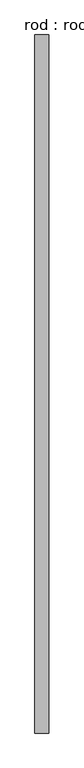
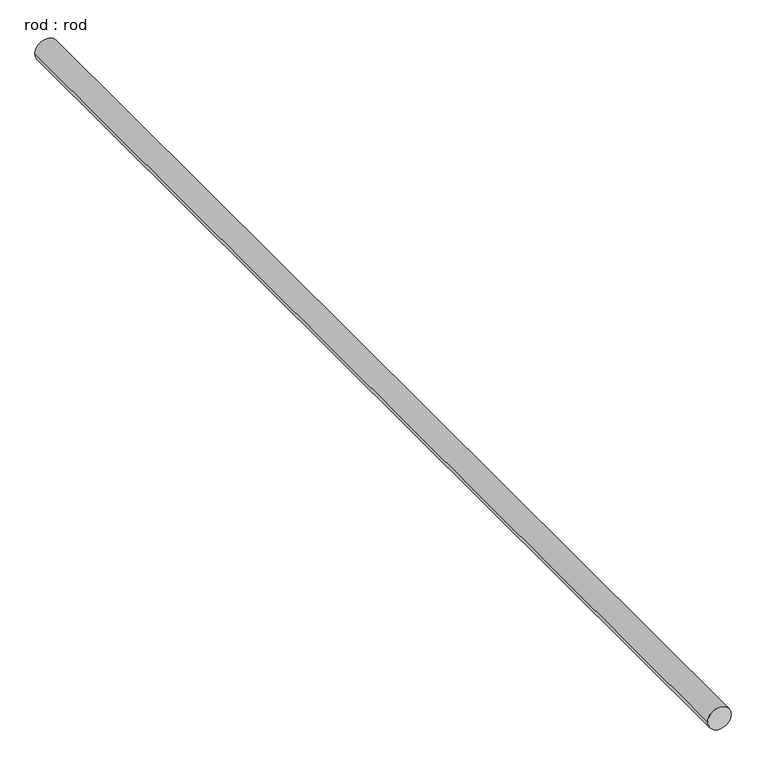
"""IFC4 building model written with IfcOpenShell, lengths in millimetres: proxy geometry, rod : rod."""

from ifc_helpers import new_model, si_unit, point, frame, frame_2d, origin, place, context, project, spatial, circle_curve, trimmed, segment, composite_curve, outline, extrude, source, transform, mapped, element, save


def rod_rod_f8a6c655(model_context):
    return source(origin(), model_context, "Body", "SweptSolid", [
        extrude(outline(composite_curve([segment(trimmed(circle_curve(frame_2d((0.0108462, 0.0)), 200.0), [point((0.0108462, 200.0))], [point((0.0108462, -200.0))], False, "CARTESIAN"), True, "CONTINUOUS"), segment(trimmed(circle_curve(frame_2d((0.0108462, 0.0)), 200.0), [point((0.0108462, -200.0))], [point((0.0108462, 200.0))], False, "CARTESIAN"), True, "CONTINUOUS")], self_intersect=False)), frame((0.0, -5907.2713847, 0.0), z_axis=(0.0, 1.0, 0.0), x_axis=(0.0, 0.0, 1.0)), (0.0, 0.0, 1.0), 20000.0),
    ])


if __name__ == "__main__":
    model = new_model("IFC4")
    model_context = context("Model", 3, world=origin())
    ifc_project = project(units=[si_unit("LENGTHUNIT", "METRE", prefix="MILLI")], contexts=[model_context])
    site = spatial("IfcSite", under=ifc_project)
    building = spatial("IfcBuilding", under=site)
    placement = place(None, origin())
    rod_rod_shape = rod_rod_f8a6c655(model_context)
    element("IfcBuildingElementProxy", 1, Name="rod : rod", ObjectType="rod : rod", at=placement, inside=building, context=model_context, shape_type="MappedRepresentation", body=[
        mapped(rod_rod_shape, transform((0.0, 0.0, 0.0), x_axis=(1.0, 0.0, 0.0), y_axis=(0.0, 1.0, 0.0), z_axis=(0.0, 0.0, 1.0))),
    ])
    save(model, "model.ifc")

# Revit data of these elements
# Type "rod : rod"
#   Default Elevation = 0
